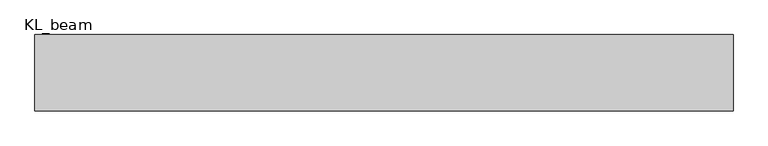
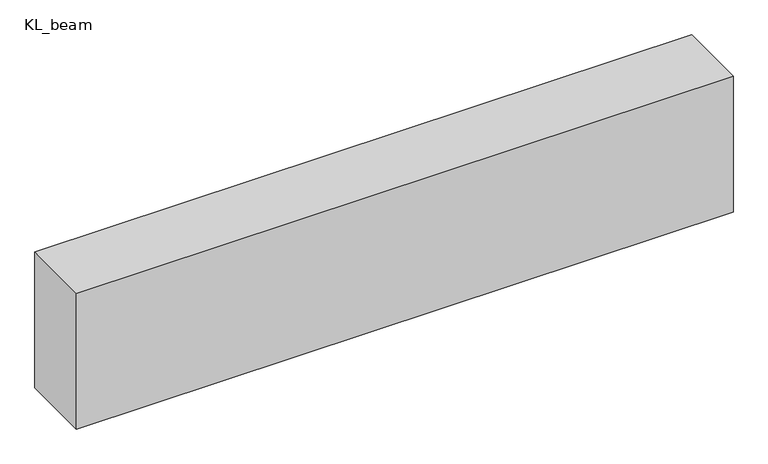
"""IFC4 building model written with IfcOpenShell, lengths in millimetres: beam geometry, 混凝土 - 矩形梁 : KL_beam."""

from ifc_helpers import new_model, si_unit, frame, origin, place, context, project, spatial, polyline, outline, extrude, source, transform, mapped, element, save


def kl_beam_000e6cef(model_context):
    return source(origin(), model_context, "Body", "SweptSolid", [
        extrude(outline(polyline([(1827.5, 200.0), (1827.5, -200.0), (-1827.5, -200.0), (-1827.5, 200.0), (1827.5, 200.0)])), frame((0.0, 0.0, -400.0), z_axis=(0.0, 0.0, 1.0), x_axis=(1.0, 0.0, 0.0)), (0.0, 0.0, 1.0), 800.0),
    ])


if __name__ == "__main__":
    model = new_model("IFC4")
    model_context = context("Model", 3, world=origin())
    ifc_project = project(units=[si_unit("LENGTHUNIT", "METRE", prefix="MILLI")], contexts=[model_context])
    site = spatial("IfcSite", under=ifc_project)
    building = spatial("IfcBuilding", under=site)
    placement = place(None, origin())
    kl_beam_shape = kl_beam_000e6cef(model_context)
    element("IfcBeam", 1, ObjectType="混凝土 - 矩形梁 : KL_beam", at=placement, inside=building, context=model_context, shape_type="MappedRepresentation", body=[
        mapped(kl_beam_shape, transform((0.0, 0.0, 0.0), x_axis=(1.0, 0.0, 0.0), y_axis=(0.0, 1.0, 0.0), z_axis=(0.0, 0.0, 1.0))),
    ])
    save(model, "model.ifc")

# Revit data of these elements
# Type "混凝土 - 矩形梁 : KL_beam"
#   Length [instance default] = 1524 mm
#   b = 400 mm
#   h = 800 mm
#   Structural Material [instance default] = 混凝土 - 现场浇注混凝土
#   Assembly Code = ""
# Element 1 (IfcBeam, "混凝土 - 矩形梁 : KL_beam")
#   Structural Material = none
# Materials
#   "混凝土 - 现场浇注混凝土": class "混凝土", colour RGB 192 192 192, transparency 0
